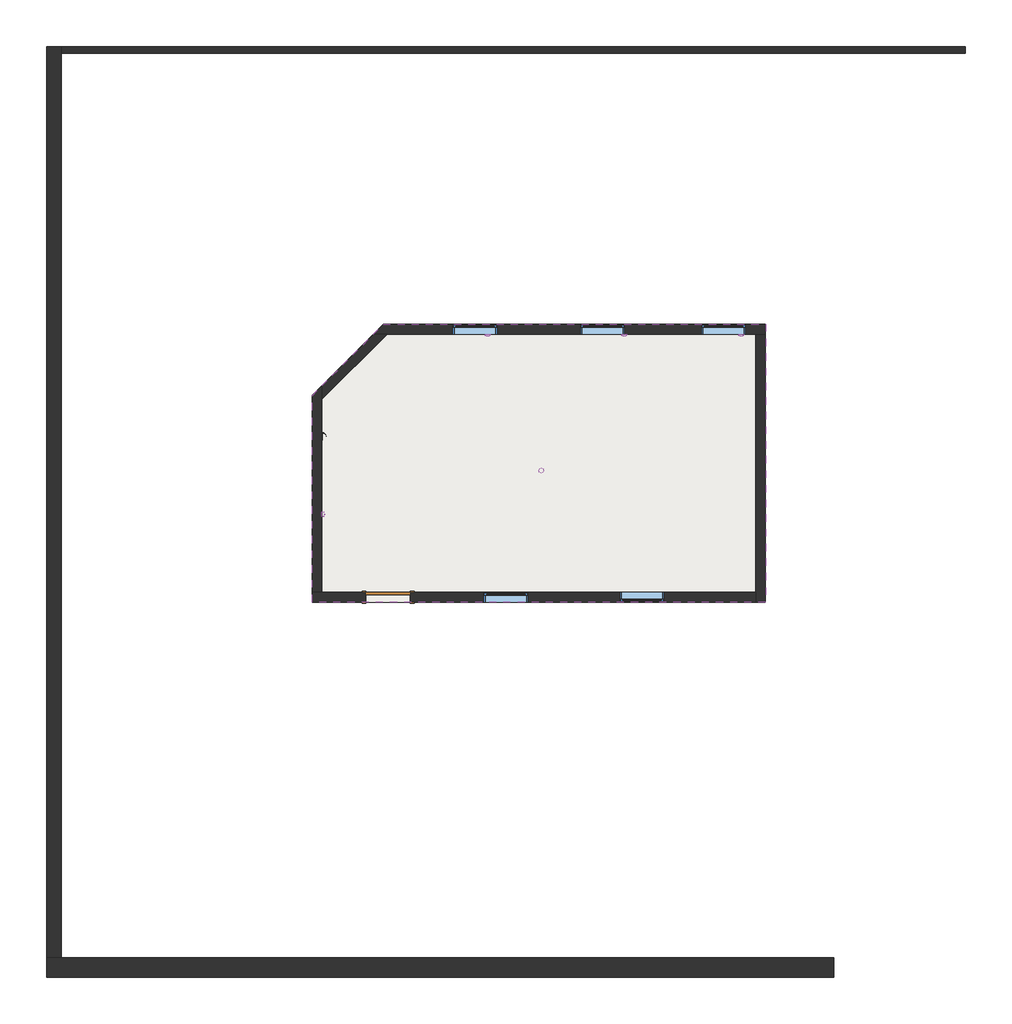
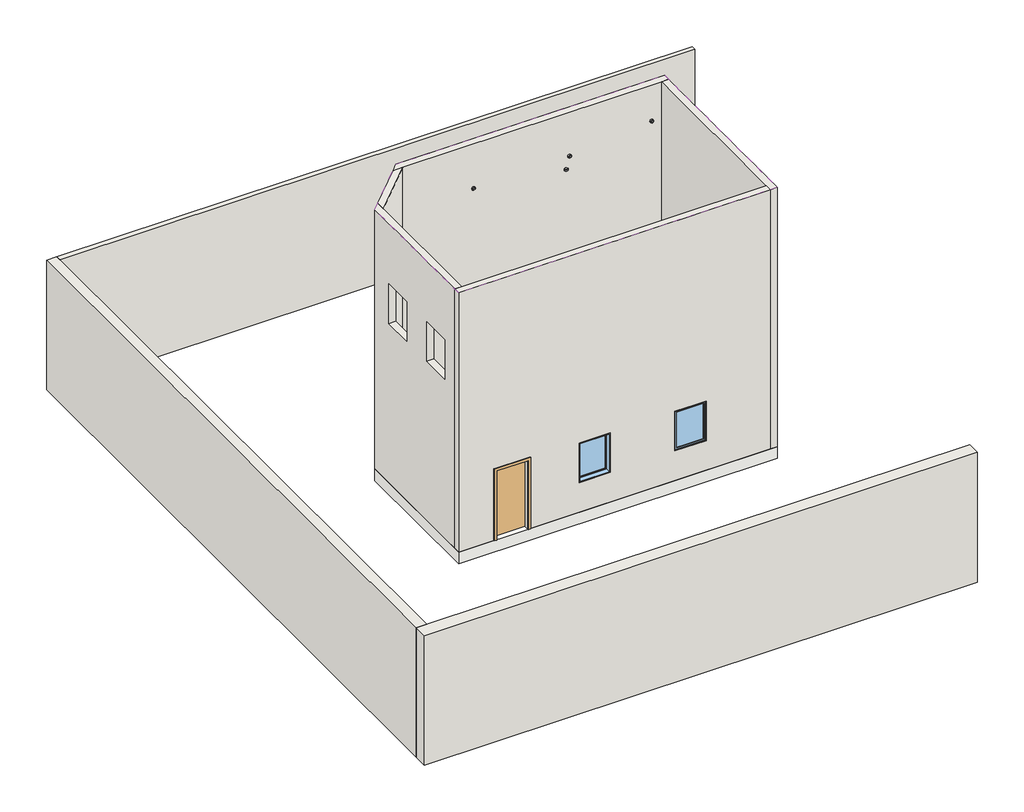
# One storey: 8 walls, 6 alarms, 5 windows, 1 door, 1 roof, 1 slab.
"""IFC4 building model written with IfcOpenShell, lengths in millimetres."""

import ifcopenshell
import ifcopenshell.guid

model = None  # the IFC model being written
_history = None  # IfcOwnerHistory: only IFC2X3 demands one
_inside = {}  # id of a spatial element -> (the spatial element, [elements in it])
_under = {}  # id of a project, library or spatial element -> (it, [spatial elements below it])
_declared = {}  # id of a project -> (the project, [libraries it declares])
_typed = {}  # id of a type object -> (the type object, [elements of that type])
_made_of = {}  # id of a material, layer set ... -> (it, [elements and type objects made of it])


def new_model(schema):
    """Start an empty IFC model of exactly this schema.

    Asked for "IFC4X3", IfcOpenShell would pick the latest addendum, in which some entities
    have other attributes; the version numbers below select the first issue.
    IFC2X3 requires an IfcOwnerHistory on every rooted entity: one is made here for all.
    """
    global model, _history
    if schema == "IFC4X3":
        model = ifcopenshell.file(schema_version=(4, 3, 0, 0))
    else:
        model = ifcopenshell.file(schema=schema)
    _inside.clear()
    _under.clear()
    _declared.clear()
    _typed.clear()
    _made_of.clear()
    _history = None
    if model.schema == "IFC2X3":
        org = make("IfcOrganization", Name="unknown")
        user = make(
            "IfcPersonAndOrganization",
            ThePerson=make("IfcPerson", FamilyName="unknown"),
            TheOrganization=org,
        )
        app = make(
            "IfcApplication",
            ApplicationDeveloper=org,
            Version="unknown",
            ApplicationFullName="unknown",
            ApplicationIdentifier="unknown",
        )
        _history = make(
            "IfcOwnerHistory",
            OwningUser=user,
            OwningApplication=app,
            ChangeAction="ADDED",
            CreationDate=0,
        )
    return model


def make(cls, **values):
    """One entity of the class cls with the attributes given. An attribute that is None is left unset."""
    return model.create_entity(
        cls, **{name: value for name, value in values.items() if value is not None}
    )


def rooted(cls, **values):
    """An entity with a GlobalId (a new one), such as an element, a storey or a relation."""
    return make(cls, GlobalId=ifcopenshell.guid.new(), OwnerHistory=_history, **values)


def si_unit(unit_type, name, prefix=None):
    """IfcSIUnit, for example si_unit("LENGTHUNIT", "METRE", prefix="MILLI")."""
    return make("IfcSIUnit", UnitType=unit_type, Prefix=prefix, Name=name)


def assignment(units):
    """IfcUnitAssignment: the units of a project."""
    return None if units is None else make("IfcUnitAssignment", Units=units)


def point(xyz):
    """IfcCartesianPoint."""
    return None if xyz is None else make("IfcCartesianPoint", Coordinates=xyz)


def direction(xyz):
    """IfcDirection."""
    return None if xyz is None else make("IfcDirection", DirectionRatios=xyz)


def frame(location, z_axis=None, x_axis=None):
    """IfcAxis2Placement3D, a coordinate frame: its origin and axes. An axis left out is left unset."""
    return make(
        "IfcAxis2Placement3D",
        Location=point(location),
        Axis=direction(z_axis),
        RefDirection=direction(x_axis),
    )


def frame_2d(location, x_axis=None):
    """IfcAxis2Placement2D, a coordinate frame in the plane: its origin and x axis."""
    return make(
        "IfcAxis2Placement2D", Location=point(location), RefDirection=direction(x_axis)
    )


def origin():
    """The frame at (0, 0, 0) with its axes left unset."""
    return frame((0.0, 0.0, 0.0))


def origin_with_axes():
    """The frame at (0, 0, 0) with the z axis (0, 0, 1) and the x axis (1, 0, 0) written out."""
    return frame((0.0, 0.0, 0.0), z_axis=(0.0, 0.0, 1.0), x_axis=(1.0, 0.0, 0.0))


def origin_2d():
    """The frame at (0, 0) in the plane with its x axis left unset."""
    return frame_2d((0.0, 0.0))


def place(relative_to, where):
    """IfcLocalPlacement: puts the frame where relative to a parent placement (None: the world)."""
    return make(
        "IfcLocalPlacement", PlacementRelTo=relative_to, RelativePlacement=where
    )


def context(
    kind, dimensions, precision=None, world=None, true_north=None, identifier=None
):
    """IfcGeometricRepresentationContext, for example the 3D "Model" context."""
    return make(
        "IfcGeometricRepresentationContext",
        ContextIdentifier=identifier,
        ContextType=kind,
        CoordinateSpaceDimension=dimensions,
        Precision=precision,
        WorldCoordinateSystem=world,
        TrueNorth=true_north,
    )


def project(units=None, contexts=None):
    """IfcProject with its units and contexts."""
    return rooted(
        "IfcProject",
        Name="project",
        RepresentationContexts=contexts,
        UnitsInContext=assignment(units),
    )


def spatial(cls, under=None, at=None, **own):
    """A site, building, storey or space (cls), placed at a placement, below another one or the project."""
    s = rooted(cls, ObjectPlacement=at, **own)
    if under is not None:
        _under.setdefault(under.id(), (under, []))[1].append(s)
    return s


def polyline(points):
    """IfcPolyline through the points."""
    return make("IfcPolyline", Points=[point(p) for p in points])


def circle_curve(where, radius):
    """IfcCircle in the frame where."""
    return make("IfcCircle", Position=where, Radius=radius)


def ellipse_curve(where, semi_axis1, semi_axis2):
    """IfcEllipse in the frame where."""
    return make(
        "IfcEllipse", Position=where, SemiAxis1=semi_axis1, SemiAxis2=semi_axis2
    )


def trimmed(basis, trim1, trim2, sense, master):
    """IfcTrimmedCurve: the piece of a basis curve between two trims."""
    return make(
        "IfcTrimmedCurve",
        BasisCurve=basis,
        Trim1=trim1,
        Trim2=trim2,
        SenseAgreement=sense,
        MasterRepresentation=master,
    )


def segment(curve, same_sense, transition):
    """IfcCompositeCurveSegment."""
    return make(
        "IfcCompositeCurveSegment",
        Transition=transition,
        SameSense=same_sense,
        ParentCurve=curve,
    )


def composite_curve(segments, self_intersect=None):
    """IfcCompositeCurve: segments joined end to end."""
    return make("IfcCompositeCurve", Segments=segments, SelfIntersect=self_intersect)


def outline(outer, holes=None, kind="AREA"):
    """IfcArbitraryClosedProfileDef: a profile drawn as a closed curve; with holes, ...WithVoids."""
    if holes is None:
        return make("IfcArbitraryClosedProfileDef", ProfileType=kind, OuterCurve=outer)
    return make(
        "IfcArbitraryProfileDefWithVoids",
        ProfileType=kind,
        OuterCurve=outer,
        InnerCurves=holes,
    )


def extrude(swept, where, along, depth):
    """IfcExtrudedAreaSolid: the profile swept, set in the frame where, extruded along a direction by depth."""
    return make(
        "IfcExtrudedAreaSolid",
        SweptArea=swept,
        Position=where,
        ExtrudedDirection=direction(along),
        Depth=depth,
    )


def faces_of(points, faces, orient=None, outer=None):
    """IfcFace entities. A face is a list of loops; a loop is a list of indices into points, from 0.

    orient and outer hold one flag for each loop. By default every Orientation is true, the
    first loop of a face is its IfcFaceOuterBound and the others are IfcFaceBound.
    """
    made = []
    for i, loops in enumerate(faces):
        bounds = []
        for j, loop in enumerate(loops):
            is_outer = j == 0 if outer is None else outer[i][j]
            bounds.append(
                make(
                    "IfcFaceOuterBound" if is_outer else "IfcFaceBound",
                    Bound=make("IfcPolyLoop", Polygon=[points[k] for k in loop]),
                    Orientation=True if orient is None else orient[i][j],
                )
            )
        made.append(make("IfcFace", Bounds=bounds))
    return made


def faceted_brep(points, faces, orient=None, outer=None, voids=None):
    """IfcFacetedBrep: a solid bounded by flat faces; with voids (closed shells), ...WithVoids."""
    shared = [point(p) for p in points]
    hull = make("IfcClosedShell", CfsFaces=faces_of(shared, faces, orient, outer))
    if voids is None:
        return make("IfcFacetedBrep", Outer=hull)
    return make(
        "IfcFacetedBrepWithVoids",
        Outer=hull,
        Voids=[
            make(cls, CfsFaces=faces_of(shared, fs, o, b)) for cls, fs, o, b in voids
        ],
    )


def shape(context_of_items, identifier, shape_type, items):
    """IfcShapeRepresentation: the items that make up one representation, for example the "Body"."""
    return make(
        "IfcShapeRepresentation",
        ContextOfItems=context_of_items,
        RepresentationIdentifier=identifier,
        RepresentationType=shape_type,
        Items=items,
    )


def source(mapping_origin, context_of_items, identifier, shape_type, items):
    """IfcRepresentationMap: a shape defined once, which mapped items show again and again."""
    return make(
        "IfcRepresentationMap",
        MappingOrigin=mapping_origin,
        MappedRepresentation=shape(context_of_items, identifier, shape_type, items),
    )


def transform(
    local_origin,
    x_axis=None,
    y_axis=None,
    z_axis=None,
    scale=None,
    scale2=None,
    scale3=None,
    uniform=True,
):
    """IfcCartesianTransformationOperator3D, or its non-uniform kind. x_axis, y_axis, z_axis: its Axis1, 2, 3."""
    if uniform:
        return make(
            "IfcCartesianTransformationOperator3D",
            Axis1=direction(x_axis),
            Axis2=direction(y_axis),
            LocalOrigin=point(local_origin),
            Scale=scale,
            Axis3=direction(z_axis),
        )
    return make(
        "IfcCartesianTransformationOperator3DnonUniform",
        Axis1=direction(x_axis),
        Axis2=direction(y_axis),
        LocalOrigin=point(local_origin),
        Scale=scale,
        Axis3=direction(z_axis),
        Scale2=scale2,
        Scale3=scale3,
    )


def mapped(mapping_source, mapping_target):
    """IfcMappedItem: shows the shape of a source again, moved by a transform."""
    return make(
        "IfcMappedItem", MappingSource=mapping_source, MappingTarget=mapping_target
    )


def made_of(thing, what):
    """Note that an element or type object is made of a material, layer set ...; save() writes the relation."""
    if what is not None:
        _made_of.setdefault(what.id(), (what, []))[1].append(thing)
    return thing


def element(
    cls,
    number,
    at=None,
    inside=None,
    cuts=None,
    type_object=None,
    material=None,
    context=None,
    identifier="Body",
    shape_type=None,
    held_by="IfcProductDefinitionShape",
    body=None,
    shapes=None,
    **own,
):
    """One element of the class cls, such as IfcWall. Its Tag is "e" and its number.

    at: its placement. inside: the storey or other place that contains it. cuts: it is an
    opening in that element (IfcRelVoidsElement). A single representation is given by context,
    identifier, shape_type and body (its items); several are given by shapes. held_by: the class
    of the entity that holds the representations. save() writes the other relations.
    """
    e = rooted(cls, Tag="e%d" % number, ObjectPlacement=at, **own)
    if body is not None:
        shapes = [shape(context, identifier, shape_type, body)]
    if shapes is not None:
        e.Representation = make(held_by, Representations=shapes)
    if inside is not None:
        _inside.setdefault(inside.id(), (inside, []))[1].append(e)
    if cuts is not None:
        rooted(
            "IfcRelVoidsElement", RelatingBuildingElement=cuts, RelatedOpeningElement=e
        )
    if type_object is not None:
        _typed.setdefault(type_object.id(), (type_object, []))[1].append(e)
    return made_of(e, material)


def aggregate(whole, parts):
    """IfcRelAggregates: a whole, such as a stair, and the parts it consists of."""
    return rooted("IfcRelAggregates", RelatingObject=whole, RelatedObjects=parts)


def save(model, path):
    """Write the relations noted so far, then the file.

    IfcRelAggregates (storeys below a building ...), IfcRelContainedInSpatialStructure (elements
    in a storey), IfcRelDefinesByType, IfcRelAssociatesMaterial and IfcRelDeclares: one each for
    every whole, place, type object, material and project.
    """
    for whole, parts in _under.values():
        aggregate(whole, parts)
    for where, things in _inside.values():
        rooted(
            "IfcRelContainedInSpatialStructure",
            RelatedElements=things,
            RelatingStructure=where,
        )
    for kind, things in _typed.values():
        rooted("IfcRelDefinesByType", RelatedObjects=things, RelatingType=kind)
    for what, things in _made_of.values():
        rooted("IfcRelAssociatesMaterial", RelatedObjects=things, RelatingMaterial=what)
    for by, libraries in _declared.values():
        rooted("IfcRelDeclares", RelatingContext=by, RelatedDefinitions=libraries)
    model.write(path)


def plane_surface(at):
    """IfcPlane: the flat surface through the origin of the frame at, square to its z axis."""
    return make("IfcPlane", Position=at)


def cylinder_surface(at, radius):
    """IfcCylindricalSurface: all points at the distance radius from the z axis of the frame at."""
    return make("IfcCylindricalSurface", Position=at, Radius=radius)


def revolved_surface(curve, axis_point, axis_direction):
    """IfcSurfaceOfRevolution: the curve turned about the line through axis_point along axis_direction."""
    return make(
        "IfcSurfaceOfRevolution",
        SweptCurve=make("IfcArbitraryOpenProfileDef", ProfileType="CURVE", Curve=curve),
        AxisPosition=make("IfcAxis1Placement", Location=point(axis_point), Axis=direction(axis_direction)),
    )


def advanced_brep(points, edges, surfaces, faces):
    """IfcAdvancedBrep: a solid bounded by faces that lie on surfaces and meet in shared edges.

    An edge is (start, end): straight between two places in points (the first is 0);
    or (start, end, curve); or (start, end, curve, False) where it runs against its curve.
    A face is (place in surfaces, loops), or (place, loops, False) where it looks against
    its surface's normal. A loop lists edges by number (the first is 1), with a minus sign
    where the edge is run from its end to its start. The first loop is the outer one.
    """
    corners = [point(p) for p in points]
    vertices = [make("IfcVertexPoint", VertexGeometry=c) for c in corners]
    made = []
    for start, end, *more in edges:
        made.append(
            make(
                "IfcEdgeCurve",
                EdgeStart=vertices[start],
                EdgeEnd=vertices[end],
                EdgeGeometry=more[0] if more else make("IfcPolyline", Points=[corners[start], corners[end]]),
                SameSense=more[1] if len(more) > 1 else True,
            )
        )
    hull = []
    for where, loops, *sense in faces:
        bounds = []
        for j, loop in enumerate(loops):
            ring = [make("IfcOrientedEdge", EdgeElement=made[abs(k) - 1], Orientation=k > 0) for k in loop]
            bounds.append(
                make(
                    "IfcFaceOuterBound" if j == 0 else "IfcFaceBound",
                    Bound=make("IfcEdgeLoop", EdgeList=ring),
                    Orientation=True,
                )
            )
        hull.append(make("IfcAdvancedFace", Bounds=bounds, FaceSurface=surfaces[where], SameSense=sense[0] if sense else True))
    return make("IfcAdvancedBrep", Outer=make("IfcClosedShell", CfsFaces=hull))


def alarm_29ba7a31(model_context):
    return source(origin(), model_context, "Body", "SolidModel", [
        advanced_brep(
        [(0.0, 0.0, 85.5), (76.0, 0.0, 9.5), (-76.0, 0.0, 9.5), (0.0, 0.0, 9.5)],
        [
            (0, 1, circle_curve(frame((0.0, 0.0, 9.5), z_axis=(0.0, 1.0, 0.0), x_axis=(1.0, 0.0, 0.0)), 76.0)),
            (1, 2, circle_curve(frame((0.0, 0.0, 9.5), z_axis=(0.0, 0.0, 1.0), x_axis=(1.0, 0.0, 0.0)), 76.0)),
            (2, 0, circle_curve(frame((0.0, 0.0, 9.5), z_axis=(0.0, 1.0, 0.0), x_axis=(-1.0, 0.0, 0.0)), 76.0)),
            (2, 1, circle_curve(frame((0.0, 0.0, 9.5), z_axis=(0.0, 0.0, 1.0), x_axis=(1.0, 0.0, 0.0)), 76.0)),
            (1, 3),
            (3, 2),
        ],
        [
            revolved_surface(trimmed(ellipse_curve(frame((0.0, 0.0, 9.5), z_axis=(0.0, -1.0, 0.0), x_axis=(1.0, 0.0, 0.0)), 76.0, 76.0), [point((76.0, 0.0, 9.5))], [point((0.0, 0.0, 85.5))], True, "CARTESIAN"), (0.0, 0.0, 2609.0581012), (0.0, 0.0, 1.0)),
            plane_surface(frame((0.0, 0.0, 9.5), z_axis=(0.0, 0.0, -1.0), x_axis=(1.0, 0.0, 0.0))),
        ],
        [
            (0, [[1, 2, 3]]),
            (0, [[-3, 4, -1]]),
            (1, [[-2, 5, 6]]),
            (1, [[-4, -6, -5]]),
        ],
    ),
        extrude(outline(composite_curve([segment(trimmed(circle_curve(origin_2d(), 76.0), [point((-76.0, 0.0))], [point((76.0, 0.0))], False, "CARTESIAN"), True, "CONTINUOUS"), segment(trimmed(circle_curve(origin_2d(), 76.0), [point((76.0, 0.0))], [point((-76.0, 0.0))], False, "CARTESIAN"), True, "CONTINUOUS")], self_intersect=False)), origin_with_axes(), (0.0, 0.0, 1.0), 9.5),
    ])


def alarm_53eb8f19(model_context):
    return source(origin(), model_context, "Body", "AdvancedBrep", [
        advanced_brep(
        [(52.0, 0.0, 0.0), (-52.0, 0.0, 0.0), (52.0, 0.0, 35.0), (-52.0, 0.0, 35.0), (-18.3847763, -18.3847763, 35.0), (0.0, 0.0, 35.0), (18.3847763, -18.3847763, 35.0), (0.0, 0.0, 60.0)],
        [
            (0, 1, circle_curve(frame((0.0, 0.0, 0.0), z_axis=(0.0, 0.0, -1.0), x_axis=(-1.0, 0.0, 0.0)), 52.0)),
            (1, 0, circle_curve(frame((0.0, 0.0, 0.0), z_axis=(0.0, 0.0, -1.0), x_axis=(-1.0, 0.0, 0.0)), 52.0)),
            (2, 3, circle_curve(frame((0.0, 0.0, 35.0), z_axis=(0.0, 0.0, 1.0), x_axis=(-1.0, 0.0, 0.0)), 52.0)),
            (3, 2, circle_curve(frame((0.0, 0.0, 35.0), z_axis=(0.0, 0.0, 1.0), x_axis=(-1.0, 0.0, 0.0)), 52.0)),
            (4, 5),
            (5, 6),
            (6, 4, circle_curve(frame((0.0, 0.0, 35.0), z_axis=(0.0, 0.0, -1.0), x_axis=(-0.7071067811865503, -0.7071067811865446, 0.0)), 26.0)),
            (1, 3),
            (2, 0),
            (4, 7),
            (7, 5),
            (7, 6),
        ],
        [
            plane_surface(frame((-52.0, 0.0, 0.0), z_axis=(0.0, 0.0, -1.0), x_axis=(0.0, 1.0, 0.0))),
            plane_surface(frame((-52.0, 0.0, 35.0), z_axis=(0.0, 0.0, 1.0), x_axis=(0.0, -1.0, 0.0))),
            cylinder_surface(frame((0.0, 0.0, 0.0), z_axis=(0.0, 0.0, 1.0), x_axis=(-1.0, 0.0, 0.0)), 52.0),
            plane_surface(frame((0.0, 0.0, 2609.0581012), z_axis=(-0.7071067811865447, 0.7071067811865505, 0.0), x_axis=(-0.7071067811865505, -0.7071067811865447, 0.0))),
            plane_surface(frame((0.0, 0.0, 2609.0581012), z_axis=(0.7071067811865515, 0.7071067811865437, 0.0), x_axis=(0.7071067811865437, -0.7071067811865515, 0.0))),
            revolved_surface(polyline([(-18.3847763, -18.3847763, 35.0), (0.0, 0.0, 60.0)]), (0.0, 0.0, 2609.0581012), (0.0, 0.0, 1.0)),
        ],
        [
            (0, [[1, 2]]),
            (1, [[3, 4], [5, 6, 7]]),
            (2, [[-2, 8, -3, 9]]),
            (2, [[-1, -9, -4, -8]]),
            (3, [[10, 11, -5]]),
            (4, [[-11, 12, -6]]),
            (5, [[-10, -7, -12]]),
        ],
    ),
        advanced_brep(
        [(26.0, 0.0, 35.0), (-26.0, 0.0, 35.0), (0.0, 0.0, 60.0), (0.0, 0.0, 35.0)],
        [
            (0, 1, circle_curve(frame((0.0, 0.0, 35.0), z_axis=(0.0, 0.0, 1.0), x_axis=(-1.0, 0.0, 0.0)), 26.0)),
            (1, 2),
            (2, 0),
            (1, 0, circle_curve(frame((0.0, 0.0, 35.0), z_axis=(0.0, 0.0, 1.0), x_axis=(-1.0, 0.0, 0.0)), 26.0)),
            (3, 1),
            (0, 3),
        ],
        [
            revolved_surface(polyline([(0.0, 0.0, 60.0), (-26.0, 0.0, 35.0)]), (0.0, 0.0, 2609.0581012), (0.0, 0.0, -1.0)),
            plane_surface(frame((0.0, 0.0, 35.0), z_axis=(0.0, 0.0, -1.0), x_axis=(-1.0, 0.0, 0.0))),
        ],
        [
            (0, [[1, 2, 3]]),
            (0, [[4, -3, -2]]),
            (1, [[5, -1, 6]]),
            (1, [[-6, -4, -5]]),
        ],
    ),
        advanced_brep(
        [(0.0, 0.0, 60.0), (-18.3847763, 18.3847763, 35.0), (0.0, 0.0, 35.0), (18.3847763, 18.3847763, 35.0)],
        [
            (0, 1),
            (1, 2),
            (2, 0),
            (2, 3),
            (3, 0),
            (1, 3, circle_curve(frame((0.0, 0.0, 35.0), z_axis=(0.0, 0.0, -1.0), x_axis=(-0.707106781186547, 0.7071067811865482, 0.0)), 26.0)),
        ],
        [
            plane_surface(frame((0.0, 0.0, 2343.8067943), z_axis=(-0.7071067811865482, -0.707106781186547, 0.0), x_axis=(-0.707106781186547, 0.7071067811865482, 0.0))),
            plane_surface(frame((0.0, 0.0, 2343.8067943), z_axis=(0.7071067811865482, -0.707106781186547, 0.0), x_axis=(0.707106781186547, 0.7071067811865482, 0.0))),
            plane_surface(frame((0.0, 0.0, 35.0), z_axis=(0.0, 0.0, -1.0000000000000002), x_axis=(-0.707106781186547, 0.7071067811865482, 0.0))),
            revolved_surface(polyline([(-18.3847763, 18.3847763, 35.0), (0.0, 0.0, 60.0)]), (0.0, 0.0, 2343.8067943), (0.0, 0.0, 1.0)),
        ],
        [
            (0, [[1, 2, 3]]),
            (1, [[4, 5, -3]]),
            (2, [[-2, 6, -4]]),
            (3, [[-6, -1, -5]]),
        ],
    ),
        advanced_brep(
        [(0.0, 0.0, 60.0), (0.0, 0.0, 35.0), (-18.3847763, 18.3847763, 35.0), (-18.3847763, -18.3847763, 35.0)],
        [
            (0, 1),
            (1, 2),
            (2, 0),
            (0, 3),
            (3, 1),
            (3, 2, circle_curve(frame((0.0, 0.0, 35.0), z_axis=(0.0, 0.0, -1.0), x_axis=(-0.707106781186547, 0.7071067811865482, 0.0)), 26.0)),
        ],
        [
            plane_surface(frame((0.0, 0.0, 2343.8067943), z_axis=(0.7071067811865482, 0.707106781186547, 0.0), x_axis=(-0.707106781186547, 0.7071067811865482, 0.0))),
            plane_surface(frame((0.0, 0.0, 2343.8067943), z_axis=(0.7071067811865459, -0.7071067811865491, 0.0), x_axis=(-0.7071067811865491, -0.7071067811865459, 0.0))),
            plane_surface(frame((0.0, 0.0, 35.0), z_axis=(0.0, 0.0, -1.0000000000000002), x_axis=(-0.707106781186547, 0.7071067811865482, 0.0))),
            revolved_surface(polyline([(-18.3847763, 18.3847763, 35.0), (0.0, 0.0, 60.0)]), (0.0, 0.0, 2343.8067943), (0.0, 0.0, 1.0)),
        ],
        [
            (0, [[1, 2, 3]]),
            (1, [[4, 5, -1]]),
            (2, [[6, -2, -5]]),
            (3, [[-3, -6, -4]]),
        ],
    ),
        advanced_brep(
        [(18.3847763, -18.3847763, 35.0), (0.0, 0.0, 60.0), (0.0, 0.0, 35.0), (18.3847763, 18.3847763, 35.0)],
        [
            (0, 1),
            (1, 2),
            (2, 0),
            (3, 2),
            (1, 3),
            (0, 3, circle_curve(frame((0.0, 0.0, 35.0), z_axis=(0.0, 0.0, 1.0), x_axis=(0.7071067811865503, -0.7071067811865446, 0.0)), 26.0)),
        ],
        [
            plane_surface(frame((0.0, 0.0, 2609.0581012), z_axis=(-0.7071067811865447, -0.7071067811865505, 0.0), x_axis=(0.7071067811865505, -0.7071067811865447, 0.0))),
            plane_surface(frame((0.0, 0.0, 2609.0581012), z_axis=(-0.7071067811865491, 0.707106781186546, 0.0), x_axis=(0.707106781186546, 0.7071067811865491, 0.0))),
            revolved_surface(polyline([(0.0, 0.0, 60.0), (18.3847763, -18.3847763, 35.0)]), (0.0, 0.0, 2609.0581012), (0.0, 0.0, -1.0)),
            plane_surface(frame((0.0, 0.0, 35.0), z_axis=(0.0, 0.0, -1.0), x_axis=(0.7071067811865505, -0.7071067811865447, 0.0))),
        ],
        [
            (0, [[1, 2, 3]]),
            (1, [[4, -2, 5]]),
            (2, [[-1, 6, -5]]),
            (3, [[-6, -3, -4]]),
        ],
    ),
    ])


def alarm_5285ee31(model_context):
    return source(origin(), model_context, "Body", "AdvancedBrep", [
        advanced_brep(
        [(-26.0, 0.0, 50.0), (26.0, 0.0, 50.0), (-52.0, 0.0, 0.0), (52.0, 0.0, 0.0), (-26.0, 0.0, 35.0), (26.0, 0.0, 35.0), (-52.0, 0.0, 35.0), (52.0, 0.0, 35.0)],
        [
            (0, 1, circle_curve(frame((0.0, 0.0, 50.0), z_axis=(0.0, 0.0, 1.0), x_axis=(1.0, 0.0, 0.0)), 26.0)),
            (1, 0, circle_curve(frame((0.0, 0.0, 50.0), z_axis=(0.0, 0.0, 1.0), x_axis=(1.0, 0.0, 0.0)), 26.0)),
            (2, 3, circle_curve(frame((0.0, 0.0, 0.0), z_axis=(0.0, 0.0, -1.0), x_axis=(1.0, 0.0, 0.0)), 52.0)),
            (3, 2, circle_curve(frame((0.0, 0.0, 0.0), z_axis=(0.0, 0.0, -1.0), x_axis=(1.0, 0.0, 0.0)), 52.0)),
            (0, 4),
            (4, 5, circle_curve(frame((0.0, 0.0, 35.0), z_axis=(0.0, 0.0, 1.0), x_axis=(1.0, 0.0, 0.0)), 26.0)),
            (5, 1),
            (5, 4, circle_curve(frame((0.0, 0.0, 35.0), z_axis=(0.0, 0.0, 1.0), x_axis=(1.0, 0.0, 0.0)), 26.0)),
            (6, 7, circle_curve(frame((0.0, 0.0, 35.0), z_axis=(0.0, 0.0, 1.0), x_axis=(1.0, 0.0, 0.0)), 52.0)),
            (7, 6, circle_curve(frame((0.0, 0.0, 35.0), z_axis=(0.0, 0.0, 1.0), x_axis=(1.0, 0.0, 0.0)), 52.0)),
            (3, 7),
            (6, 2),
        ],
        [
            plane_surface(frame((26.0, 0.0, 50.0), z_axis=(0.0, 0.0, 1.0), x_axis=(0.0, 1.0, 0.0))),
            plane_surface(frame((26.0, 0.0, 0.0), z_axis=(0.0, 0.0, -1.0), x_axis=(0.0, -1.0, 0.0))),
            cylinder_surface(origin_with_axes(), 26.0),
            plane_surface(frame((52.0, 0.0, 35.0), z_axis=(0.0, 0.0, 1.0), x_axis=(0.0, 1.0, 0.0))),
            cylinder_surface(origin_with_axes(), 52.0),
        ],
        [
            (0, [[1, 2]]),
            (1, [[3, 4]]),
            (2, [[-1, 5, 6, 7]]),
            (2, [[-2, -7, 8, -5]]),
            (3, [[9, 10], [-6, -8]]),
            (4, [[-4, 11, -9, 12]]),
            (4, [[-3, -12, -10, -11]]),
        ],
    ),
    ])


def door_0915_x_2134mm_6a9e8738(model_context):
    return source(origin(), model_context, "Body", "SweptSolid", [
        extrude(outline(polyline([(2210.0, -533.5), (0.0, -533.5), (0.0, -457.5), (2134.0, -457.5), (2134.0, 457.5), (0.0, 457.5), (0.0, 533.5), (2210.0, 533.5), (2210.0, -533.5)])), frame((0.0, 100.0, 0.0), z_axis=(0.0, 1.0, 0.0), x_axis=(0.0, 0.0, 1.0)), (0.0, 0.0, 1.0), 25.0),
        extrude(outline(polyline([(2210.0, 533.5), (2210.0, -533.5), (0.0, -533.5), (0.0, -457.5), (2134.0, -457.5), (2134.0, 457.5), (0.0, 457.5), (0.0, 533.5), (2210.0, 533.5)])), frame((0.0, -125.0, 0.0), z_axis=(0.0, 1.0, 0.0), x_axis=(0.0, 0.0, 1.0)), (0.0, 0.0, 1.0), 25.0),
        extrude(outline(polyline([(457.5, 49.0), (-457.5, 49.0), (-457.5, 100.0), (457.5, 100.0), (457.5, 49.0)])), origin_with_axes(), (0.0, 0.0, 1.0), 2134.0),
    ])


def window_0915_x_1220mm_488fb2fb(model_context):
    return source(origin(), model_context, "Body", "SweptSolid", [
        extrude(outline(polyline([(-394.5, 78.0), (394.5, 78.0), (394.5, 66.0), (-394.5, 66.0), (-394.5, 78.0)])), frame((0.0, 0.0, 978.0), z_axis=(0.0, 0.0, 1.0), x_axis=(1.0, 0.0, 0.0)), (0.0, 0.0, 1.0), 1094.0),
        extrude(outline(polyline([(2116.0, -438.5), (934.0, -438.5), (934.0, 438.5), (2116.0, 438.5), (2116.0, -438.5)]), holes=[polyline([(2072.0, -394.5), (2072.0, 394.5), (978.0, 394.5), (978.0, -394.5), (2072.0, -394.5)])]), frame((0.0, 50.0, 0.0), z_axis=(0.0, 1.0, 0.0), x_axis=(0.0, 0.0, 1.0)), (0.0, 0.0, 1.0), 44.0),
        extrude(outline(polyline([(2135.0, -457.5), (915.0, -457.5), (915.0, 457.5), (2135.0, 457.5), (2135.0, -457.5)]), holes=[polyline([(2116.0, -438.5), (2116.0, 438.5), (934.0, 438.5), (934.0, -438.5), (2116.0, -438.5)])]), frame((0.0, 50.0, 0.0), z_axis=(0.0, 1.0, 0.0), x_axis=(0.0, 0.0, 1.0)), (0.0, 0.0, 1.0), 63.0),
        extrude(outline(polyline([(2135.0, -457.5), (915.0, -457.5), (915.0, 457.5), (2135.0, 457.5), (2135.0, -457.5)]), holes=[polyline([(2103.0, -425.5), (2103.0, 425.5), (947.0, 425.5), (947.0, -425.5), (2103.0, -425.5)])]), frame((0.0, -87.0, 0.0), z_axis=(0.0, 1.0, 0.0), x_axis=(0.0, 0.0, 1.0)), (0.0, 0.0, 1.0), 137.0),
    ])


model = new_model("IFC4")

# Units and contexts
model_context = context("Model", 3, world=origin())
ifc_project = project(units=[si_unit("LENGTHUNIT", "METRE", prefix="MILLI")], contexts=[model_context])

# Site, building, storey
site = spatial("IfcSite", under=ifc_project)
building = spatial("IfcBuilding", under=site)
storey = spatial("IfcBuildingStorey", under=building, Name="标高 1", Elevation=0.0)

# Alarms
placement = place(None, origin())
alarm_shape = alarm_29ba7a31(model_context)
element("IfcAlarm", 1, ObjectType="报警闪灯 : 标准", at=placement, inside=storey, context=model_context, shape_type="MappedRepresentation", body=[
    mapped(alarm_shape, transform((-7480.1449608, 2535.4590579, 1200.0), x_axis=(0.0, 1.0, 0.0), y_axis=(0.0, 0.0, 1.0), z_axis=(1.0, 0.0, 0.0))),
])
alarm_2_shape = alarm_53eb8f19(model_context)
element("IfcAlarm", 2, ObjectType="电子感温探测器 : 防爆型", at=placement, inside=storey, context=model_context, shape_type="MappedRepresentation", body=[
    mapped(alarm_2_shape, transform((-7480.1449608, 935.4590579, 6895.7404718), x_axis=(0.0, 1.0, 0.0), y_axis=(0.0, 0.0, 1.0), z_axis=(1.0, 0.0, 0.0))),
])
alarm_3_shape = alarm_5285ee31(model_context)
element("IfcAlarm", 3, ObjectType="光电感烟探测器 : 点型", at=placement, inside=storey, context=model_context, shape_type="MappedRepresentation", body=[
    mapped(alarm_3_shape, transform((-2980.1449608, 1835.4590579, 8508.5629281), x_axis=(1.0, 0.0, 0.0), y_axis=(0.0, 1.0, 0.0), z_axis=(0.0, 0.0, 1.0))),
])
element("IfcAlarm", 4, ObjectType="光电感烟探测器 : 点型", at=placement, inside=storey, context=model_context, shape_type="MappedRepresentation", body=[
    mapped(alarm_3_shape, transform((-4080.1449608, 4635.4590579, 6642.6361081), x_axis=(1.0, 0.0, 0.0), y_axis=(0.0, 0.0, 1.0), z_axis=(0.0, -1.0, 0.0))),
])
element("IfcAlarm", 5, ObjectType="光电感烟探测器 : 点型", at=placement, inside=storey, context=model_context, shape_type="MappedRepresentation", body=[
    mapped(alarm_3_shape, transform((-1280.1449608, 4635.4590579, 6660.302945), x_axis=(1.0, 0.0, 0.0), y_axis=(0.0, 0.0, 1.0), z_axis=(0.0, -1.0, 0.0))),
])
element("IfcAlarm", 6, ObjectType="光电感烟探测器 : 点型", at=placement, inside=storey, context=model_context, shape_type="MappedRepresentation", body=[
    mapped(alarm_3_shape, transform((1119.8550392, 4635.4590579, 6900.0711466), x_axis=(1.0, 0.0, 0.0), y_axis=(0.0, 0.0, 1.0), z_axis=(0.0, -1.0, 0.0))),
])

# Door
door_0915_x_2134mm_shape = door_0915_x_2134mm_6a9e8738(model_context)
element("IfcDoor", 7, ObjectType="单扇 - 与墙齐 : 0915 x 2134mm", at=placement, inside=storey, context=model_context, shape_type="MappedRepresentation", body=[
    mapped(door_0915_x_2134mm_shape, transform((-6122.6449608, -764.5409421, 0.0), x_axis=(1.0, 0.0, 0.0), y_axis=(0.0, 1.0, 0.0), z_axis=(0.0, 0.0, 1.0))),
])

# Roof
element("IfcRoof", 8, ObjectType="钢筋托梁 - 钢面板 - EPDM 薄膜", at=placement, inside=storey, context=model_context, shape_type="SweptSolid", body=[
    extrude(outline(polyline([(-7683.1449608, 3373.8804141), (-6218.566317, 4838.4590579), (1622.8550392, 4838.4590579), (1622.8550392, -867.5409421), (-7683.1449608, -867.5409421), (-7683.1449608, 3373.8804141)])), frame((0.0, 0.0, 8003.5629281), z_axis=(0.0, 0.0, 1.0), x_axis=(1.0, 0.0, 0.0)), (0.0, 0.0, 1.0), 505.0),
])

# Slab
element("IfcSlab", 9, ObjectType="混凝土 - 商用 362mm", at=placement, inside=storey, context=model_context, shape_type="SweptSolid", body=[
    extrude(outline(polyline([(-6221.566317, 4835.4590579), (1619.8550392, 4835.4590579), (1619.8550392, -864.5409421), (-7680.1449608, -864.5409421), (-7680.1449608, 3376.8804141), (-6221.566317, 4835.4590579)])), frame((0.0, 0.0, -362.0), z_axis=(0.0, 0.0, 1.0), x_axis=(1.0, 0.0, 0.0)), (0.0, 0.0, 1.0), 362.0),
])

# Walls
element("IfcWall", 10, ObjectType="常规 - 200mm", at=placement, inside=storey, context=model_context, shape_type="Brep", body=[
    faceted_brep([(-6421.566317, 4635.4590579, 0.0), (-6138.7236046, 4635.4590579, 0.0), (1419.8550392, 4635.4590579, 0.0), (1619.8550392, 4635.4590579, 0.0), (1619.8550392, 4635.4590579, 8000.0), (1419.8550392, 4635.4590579, 8000.0), (-6138.7236046, 4635.4590579, 8000.0), (-6421.566317, 4635.4590579, 8000.0), (-4795.1449608, 4635.4590579, 915.0), (-4795.1449608, 4635.4590579, 2135.0), (-3880.1449608, 4635.4590579, 2135.0), (-3880.1449608, 4635.4590579, 915.0), (-2180.1449608, 4635.4590579, 915.0), (-2180.1449608, 4635.4590579, 2135.0), (-1265.1449608, 4635.4590579, 2135.0), (-1265.1449608, 4635.4590579, 915.0), (304.8550392, 4635.4590579, 915.0), (304.8550392, 4635.4590579, 2135.0), (1219.8550392, 4635.4590579, 2135.0), (1219.8550392, 4635.4590579, 915.0), (1619.8550392, 4835.4590579, 0.0), (-6221.566317, 4835.4590579, 0.0), (-6221.566317, 4835.4590579, 8000.0), (1619.8550392, 4835.4590579, 8000.0), (-4795.1449608, 4835.4590579, 915.0), (-3880.1449608, 4835.4590579, 915.0), (-3880.1449608, 4835.4590579, 2135.0), (-4795.1449608, 4835.4590579, 2135.0), (-2180.1449608, 4835.4590579, 915.0), (-1265.1449608, 4835.4590579, 915.0), (-1265.1449608, 4835.4590579, 2135.0), (-2180.1449608, 4835.4590579, 2135.0), (304.8550392, 4835.4590579, 2135.0), (304.8550392, 4835.4590579, 915.0), (1219.8550392, 4835.4590579, 915.0), (1219.8550392, 4835.4590579, 2135.0)], [[[0, 1, 2, 3, 4, 5, 6, 7], [8, 9, 10, 11], [12, 13, 14, 15], [16, 17, 18, 19]], [[20, 21, 22, 23], [24, 25, 26, 27], [28, 29, 30, 31], [32, 33, 34, 35]], [[3, 2, 1, 0, 21, 20]], [[7, 6, 5, 4, 23, 22]], [[4, 3, 20, 23]], [[0, 7, 22, 21]], [[9, 8, 24, 27]], [[10, 9, 27, 26]], [[11, 10, 26, 25]], [[8, 11, 25, 24]], [[13, 12, 28, 31]], [[14, 13, 31, 30]], [[15, 14, 30, 29]], [[12, 15, 29, 28]], [[16, 33, 32, 17]], [[17, 32, 35, 18]], [[18, 35, 34, 19]], [[33, 16, 19, 34]]]),
])
element("IfcWall", 11, ObjectType="常规 - 200mm", at=placement, inside=storey, context=model_context, shape_type="Brep", body=[
    faceted_brep([(1419.8550392, 4635.4590579, 0.0), (1419.8550392, -664.5409421, 0.0), (1419.8550392, -864.5409421, 0.0), (1419.8550392, -864.5409421, 8000.0), (1419.8550392, -664.5409421, 8000.0), (1419.8550392, 4635.4590579, 8000.0), (1619.8550392, 4635.4590579, 0.0), (1619.8550392, 4635.4590579, 8000.0), (1619.8550392, -864.5409421, 8000.0), (1619.8550392, -864.5409421, 0.0)], [[[0, 1, 2, 3, 4, 5]], [[6, 7, 8, 9]], [[2, 1, 0, 6, 9]], [[5, 4, 3, 8, 7]], [[0, 5, 7, 6]], [[3, 2, 9, 8]]]),
])
element("IfcWall", 12, ObjectType="常规 - 200mm", at=placement, inside=storey, context=model_context, shape_type="Brep", body=[
    faceted_brep([(1419.8550392, -664.5409421, 0.0), (-5665.1449608, -664.5409421, 0.0), (-5665.1449608, -664.5409421, 2134.0), (-6580.1449608, -664.5409421, 2134.0), (-6580.1449608, -664.5409421, 0.0), (-7480.1449608, -664.5409421, 0.0), (-7680.1449608, -664.5409421, 0.0), (-7680.1449608, -664.5409421, 8000.0), (-7480.1449608, -664.5409421, 8000.0), (1419.8550392, -664.5409421, 8000.0), (-4165.1449608, -664.5409421, 915.0), (-3250.1449608, -664.5409421, 915.0), (-3250.1449608, -664.5409421, 2135.0), (-4165.1449608, -664.5409421, 2135.0), (-457.6449608, -664.5409421, 915.0), (-457.6449608, -664.5409421, 2135.0), (-1372.6449608, -664.5409421, 2135.0), (-1372.6449608, -664.5409421, 915.0), (-5665.1449608, -864.5409421, 2134.0), (-5665.1449608, -864.5409421, 0.0), (1419.8550392, -864.5409421, 0.0), (1419.8550392, -864.5409421, 8000.0), (-7680.1449608, -864.5409421, 8000.0), (-7680.1449608, -864.5409421, 0.0), (-6580.1449608, -864.5409421, 0.0), (-6580.1449608, -864.5409421, 2134.0), (-4165.1449608, -864.5409421, 915.0), (-4165.1449608, -864.5409421, 2135.0), (-3250.1449608, -864.5409421, 2135.0), (-3250.1449608, -864.5409421, 915.0), (-457.6449608, -864.5409421, 2135.0), (-457.6449608, -864.5409421, 915.0), (-1372.6449608, -864.5409421, 915.0), (-1372.6449608, -864.5409421, 2135.0)], [[[0, 1, 2, 3, 4, 5, 6, 7, 8, 9], [10, 11, 12, 13], [14, 15, 16, 17]], [[18, 19, 20, 21, 22, 23, 24, 25], [26, 27, 28, 29], [30, 31, 32, 33]], [[24, 23, 6, 5, 4]], [[20, 19, 1, 0]], [[9, 8, 7, 22, 21]], [[0, 9, 21, 20]], [[7, 6, 23, 22]], [[2, 1, 19, 18]], [[3, 2, 18, 25]], [[4, 3, 25, 24]], [[27, 26, 10, 13]], [[28, 27, 13, 12]], [[29, 28, 12, 11]], [[26, 29, 11, 10]], [[14, 31, 30, 15]], [[15, 30, 33, 16]], [[16, 33, 32, 17]], [[31, 14, 17, 32]]]),
])
element("IfcWall", 13, ObjectType="常规 - 200mm", at=placement, inside=storey, context=model_context, shape_type="Brep", body=[
    faceted_brep([(-7480.1449608, -664.5409421, 0.0), (-7480.1449608, 3294.0377016, 0.0), (-7480.1449608, 3576.8804141, 0.0), (-7480.1449608, 3576.8804141, 8000.0), (-7480.1449608, 3294.0377016, 8000.0), (-7480.1449608, -664.5409421, 8000.0), (-7480.1449608, -164.5409421, 4915.0), (-7480.1449608, -164.5409421, 6135.0), (-7480.1449608, 750.4590579, 6135.0), (-7480.1449608, 750.4590579, 4915.0), (-7480.1449608, 1750.4590579, 4915.0), (-7480.1449608, 1750.4590579, 6135.0), (-7480.1449608, 2665.4590579, 6135.0), (-7480.1449608, 2665.4590579, 4915.0), (-7680.1449608, -664.5409421, 0.0), (-7680.1449608, -664.5409421, 8000.0), (-7680.1449608, 3376.8804141, 8000.0), (-7680.1449608, 3376.8804141, 0.0), (-7680.1449608, -164.5409421, 4915.0), (-7680.1449608, 750.4590579, 4915.0), (-7680.1449608, 750.4590579, 6135.0), (-7680.1449608, -164.5409421, 6135.0), (-7680.1449608, 1750.4590579, 4915.0), (-7680.1449608, 2665.4590579, 4915.0), (-7680.1449608, 2665.4590579, 6135.0), (-7680.1449608, 1750.4590579, 6135.0)], [[[0, 1, 2, 3, 4, 5], [6, 7, 8, 9], [10, 11, 12, 13]], [[14, 15, 16, 17], [18, 19, 20, 21], [22, 23, 24, 25]], [[2, 1, 0, 14, 17]], [[5, 4, 3, 16, 15]], [[0, 5, 15, 14]], [[3, 2, 17, 16]], [[7, 6, 18, 21]], [[8, 7, 21, 20]], [[9, 8, 20, 19]], [[6, 9, 19, 18]], [[11, 10, 22, 25]], [[12, 11, 25, 24]], [[13, 12, 24, 23]], [[10, 13, 23, 22]]]),
])
element("IfcWall", 14, ObjectType="常规 - 200mm", at=placement, inside=storey, context=model_context, shape_type="SweptSolid", body=[
    extrude(outline(polyline([(-6138.7236046, 4635.4590579), (-7480.1449608, 3294.0377016), (-7480.1449608, 3576.8804141), (-6421.566317, 4635.4590579), (-6138.7236046, 4635.4590579)])), origin_with_axes(), (0.0, 0.0, 1.0), 8000.0),
])
element("IfcWall", 15, ObjectType="常规 - 140mm 砌体", at=placement, inside=storey, context=model_context, shape_type="SweptSolid", body=[
    extrude(outline(polyline([(5719.8550392, 10395.4590579), (-12830.1449608, 10395.4590579), (-12830.1449608, 10535.4590579), (5719.8550392, 10535.4590579), (5719.8550392, 10395.4590579)])), origin_with_axes(), (0.0, 0.0, 1.0), 4000.0),
])
element("IfcWall", 16, ObjectType="常规 - 225mm 砌体", at=placement, inside=storey, context=model_context, shape_type="Brep", body=[
    faceted_brep([(3019.8550392, -8164.5409421, 0.0), (-12830.1449608, -8164.5409421, 0.0), (-13130.1449608, -8164.5409421, 0.0), (-13130.1449608, -8164.5409421, 4000.0), (-12830.1449608, -8164.5409421, 4000.0), (3019.8550392, -8164.5409421, 4000.0), (3019.8550392, -8564.5409421, 0.0), (3019.8550392, -8564.5409421, 4000.0), (-13130.1449608, -8564.5409421, 4000.0), (-13130.1449608, -8564.5409421, 0.0)], [[[0, 1, 2, 3, 4, 5]], [[6, 7, 8, 9]], [[3, 2, 9, 8]], [[2, 1, 0, 6, 9]], [[5, 4, 3, 8, 7]], [[0, 5, 7, 6]]]),
])
element("IfcWall", 17, ObjectType="挡土墙 - 300mm 混凝土", at=placement, inside=storey, context=model_context, shape_type="Brep", body=[
    faceted_brep([(-12830.1449608, -8164.5409421, 0.0), (-12830.1449608, 10395.4590579, 0.0), (-12830.1449608, 10535.4590579, 0.0), (-12830.1449608, 10535.4590579, 4000.0), (-12830.1449608, 10395.4590579, 4000.0), (-12830.1449608, -8164.5409421, 4000.0), (-13130.1449608, -8164.5409421, 0.0), (-13130.1449608, -8164.5409421, 4000.0), (-13130.1449608, 10535.4590579, 4000.0), (-13130.1449608, 10535.4590579, 0.0)], [[[0, 1, 2, 3, 4, 5]], [[6, 7, 8, 9]], [[0, 5, 7, 6]], [[2, 1, 0, 6, 9]], [[5, 4, 3, 8, 7]], [[3, 2, 9, 8]]]),
])

# Windows
window_0915_x_1220mm_shape = window_0915_x_1220mm_488fb2fb(model_context)
element("IfcWindow", 18, ObjectType="固定 : 0915 x 1220mm", at=placement, inside=storey, context=model_context, shape_type="MappedRepresentation", body=[
    mapped(window_0915_x_1220mm_shape, transform((-3707.6449608, -777.5409421, 0.0), x_axis=(1.0, 0.0, 0.0), y_axis=(0.0, 1.0, 0.0), z_axis=(0.0, 0.0, 1.0))),
])
element("IfcWindow", 19, ObjectType="固定 : 0915 x 1220mm", at=placement, inside=storey, context=model_context, shape_type="MappedRepresentation", body=[
    mapped(window_0915_x_1220mm_shape, transform((-915.1449608, -751.5409421, 0.0), x_axis=(-1.0, 0.0, 0.0), y_axis=(0.0, -1.0, 0.0), z_axis=(0.0, 0.0, 1.0))),
])
element("IfcWindow", 20, ObjectType="固定 : 0915 x 1220mm", at=placement, inside=storey, context=model_context, shape_type="MappedRepresentation", body=[
    mapped(window_0915_x_1220mm_shape, transform((-4337.6449608, 4722.4590579, 0.0), x_axis=(1.0, 0.0, 0.0), y_axis=(0.0, 1.0, 0.0), z_axis=(0.0, 0.0, 1.0))),
])
element("IfcWindow", 21, ObjectType="固定 : 0915 x 1220mm", at=placement, inside=storey, context=model_context, shape_type="MappedRepresentation", body=[
    mapped(window_0915_x_1220mm_shape, transform((-1722.6449608, 4722.4590579, 0.0), x_axis=(1.0, 0.0, 0.0), y_axis=(0.0, 1.0, 0.0), z_axis=(0.0, 0.0, 1.0))),
])
element("IfcWindow", 22, ObjectType="固定 : 0915 x 1220mm", at=placement, inside=storey, context=model_context, shape_type="MappedRepresentation", body=[
    mapped(window_0915_x_1220mm_shape, transform((762.3550392, 4722.4590579, 0.0), x_axis=(1.0, 0.0, 0.0), y_axis=(0.0, 1.0, 0.0), z_axis=(0.0, 0.0, 1.0))),
])

save(model, "model.ifc")

# Revit data of these elements
# Project information
#   项目发布日期 = "出图日期"
#   项目状态 = "项目状态"
#   客户姓名 = "所有者"
#   项目地址 = "请在此处输入地址"
#   项目名称 = "项目名称"
#   项目编号 = "项目编号"
# Type "报警闪灯 : 标准"
#   半径 = 76 mm
#   高度 = 9.5 mm
#   直径 = 152 mm
#   Default Elevation = 1200 mm
#   材质 = none
# Type "电子感温探测器 : 防爆型"
#   半径 2 = 52 mm
#   半径 1 = 26 mm
#   长度 3 = 18.385 mm
#   长度 2 = 22.517 mm
#   长度 1 = 36.77 mm
#   高度 4 = 1.562 mm
#   高度 3 = 17.5 mm
#   高度 2 = 25 mm
#   高度 1 = 35 mm
#   Default Elevation = 1200 mm
#   可见性 1 = no
#   可见性 2 = yes
#   材质 = none
# Type "光电感烟探测器 : 点型"
#   半径 3 = 36.77 mm
#   半径 2 = 52 mm
#   半径 1 = 26 mm
#   高度 2 = 15 mm
#   高度 1 = 35 mm
#   Default Elevation = 1200 mm
#   可见性 2 = no
#   可见性 1 = yes
#   材质 = none
# Type "单扇 - 与墙齐 : 0915 x 2134mm"
#   Type Mark = "10"
#   Construction Type Id = "MDOOR"
#   Analytic Construction = "金属"
#   Thickness = 51 mm
#   Heat Transfer Coefficient (U) = 3.7021 W/(m²·K)
#   Height = 2134 mm
#   贴面投影外部 = 25 mm
#   贴面投影内部 = 25 mm
#   贴面宽度 = 76 mm
#   Width = 915 mm
#   Function = 0
#   门材质 = 门 - 嵌板
#   框架材质 = 门 - 框架
#   Visual Light Transmittance = 0
#   Solar Heat Gain Coefficient = 0
#   Function = (empty or 0)
#   Wall Closure = (empty or 0)
# Type "钢筋托梁 - 钢面板 - EPDM 薄膜"
#   Layers, outside or top first: 5 mm "屋顶材料 - EPDM 薄膜" (function 4); 50 mm "刚性隔热层" (function 3); 50 mm "金属 - 面板" (function 1); 400 mm "结构 - 钢筋托梁层" (function 1)
# Type "混凝土 - 商用 362mm"
#   Function = 0
#   Layers, outside or top first: 200 mm "混凝土 - 现场浇注" (function 1); 0 mm "防湿" (function 100); 12 mm "沙" (function 0); 150 mm "场地 - 碎石" (function 0)
# Type "常规 - 200mm"
#   Layers, outside or top first: 200 mm no material (function 1)
# Type "常规 - 140mm 砌体"
#   Layers, outside or top first: 140 mm "混凝土砌块" (function 1)
# Type "常规 - 225mm 砌体"
#   Layers, outside or top first: 400 mm "混凝土砌块" (function 1)
# Type "挡土墙 - 300mm 混凝土"
#   Layers, outside or top first: 300 mm "混凝土 - 现场浇注" (function 1)
# Type "固定 : 0915 x 1220mm"
#   Type Mark = "15"
#   Construction Type Id = "GSP4R"
#   Analytic Construction = "1/8 英寸 Pilkington 单层玻璃"
#   Visual Light Transmittance = 0.9
#   Solar Heat Gain Coefficient = 0.78
#   Heat Transfer Coefficient (U) = 3.6886 W/(m²·K)
#   Height = 1220 mm
#   默认窗台高度 = 915 mm
#   Width = 915 mm
#   窗嵌入 = 19 mm
#   框架外部材质 = 窗扇
#   框架内部材质 = 窗扇
#   玻璃嵌板材质 = 玻璃
#   窗扇 = 窗扇
#   Wall Closure = (empty or 0)
# Element 1 (IfcAlarm, "报警闪灯 : 标准")
#   Mark = "1"
#   Phase Created = 阶段 1
# Element 2 (IfcAlarm, "电子感温探测器 : 防爆型")
#   Mark = "8"
#   Phase Created = 阶段 1
# Element 3 (IfcAlarm, "光电感烟探测器 : 点型")
#   Mark = "4"
#   Phase Created = 阶段 1
# Element 4 (IfcAlarm, "光电感烟探测器 : 点型")
#   Mark = "5"
#   Phase Created = 阶段 1
# Element 5 (IfcAlarm, "光电感烟探测器 : 点型")
#   Mark = "6"
#   Phase Created = 阶段 1
# Element 6 (IfcAlarm, "光电感烟探测器 : 点型")
#   Mark = "7"
#   Phase Created = 阶段 1
# Element 7 (IfcDoor, "单扇 - 与墙齐 : 0915 x 2134mm")
#   Phase Created = 阶段 1
#   Materials on its faces: "门 - 框架", "门 - 嵌板"
# Element 8 (IfcRoof, "钢筋托梁 - 钢面板 - EPDM 薄膜")
#   built-in parameter 1001705 = 27.9152 (stored number, unit not read)
#   built-in parameter 1001701 = 26.2584 (stored number, unit not read)
#   built-in parameter 1001710 = 33615
#   Phase Created = 阶段 1
#   Materials on its faces: "结构 - 钢筋托梁层", "屋顶材料 - EPDM 薄膜"
# Element 9 (IfcSlab, "混凝土 - 商用 362mm")
#   built-in parameter 1001955 = 0.785398 (stored number, unit not read)
#   Height Offset From Level = 0 mm
#   Phase Created = 阶段 1
#   Materials on its faces: "场地 - 碎石", "混凝土 - 现场浇注"
# Elements 10, 11, 12, 13, 14 (IfcWall, "常规 - 200mm")
#   Top Offset = 0 mm
#   Base Offset = 0 mm
#   Unconnected Height = 8000 mm
#   wall height = 8000 mm
#   Phase Created = 阶段 1
#   Base Constraint = 标高 1
#   Materials on its faces: "默认墙"
# Element 15 (IfcWall, "常规 - 140mm 砌体")
#   Top Offset = 0 mm
#   Base Offset = 0 mm
#   Unconnected Height = 4000 mm
#   wall height = 4000 mm
#   Phase Created = 阶段 1
#   Base Constraint = 标高 1
#   Materials on its faces: "混凝土砌块"
# Element 16 (IfcWall, "常规 - 225mm 砌体")
#   Top Offset = 0 mm
#   Base Offset = 0 mm
#   Unconnected Height = 4000 mm
#   wall height = 4000 mm
#   Phase Created = 阶段 1
#   Base Constraint = 标高 1
#   Materials on its faces: "混凝土砌块", "混凝土 - 现场浇注"
# Element 17 (IfcWall, "挡土墙 - 300mm 混凝土")
#   Top Offset = 0 mm
#   Base Offset = 0 mm
#   Unconnected Height = 4000 mm
#   wall height = 4000 mm
#   Phase Created = 阶段 1
#   Base Constraint = 标高 1
#   Materials on its faces: "混凝土 - 现场浇注", "混凝土砌块"
# Element 18 (IfcWindow, "固定 : 0915 x 1220mm")
#   Mark = "1"
#   Phase Created = 阶段 1
#   Materials on its faces: "窗扇", "玻璃"
# Element 19 (IfcWindow, "固定 : 0915 x 1220mm")
#   Mark = "2"
#   Phase Created = 阶段 1
#   Materials on its faces: "窗扇", "玻璃"
# Element 20 (IfcWindow, "固定 : 0915 x 1220mm")
#   Mark = "3"
#   Phase Created = 阶段 1
#   Materials on its faces: "窗扇", "玻璃"
# Element 21 (IfcWindow, "固定 : 0915 x 1220mm")
#   Mark = "4"
#   Phase Created = 阶段 1
#   Materials on its faces: "窗扇", "玻璃"
# Element 22 (IfcWindow, "固定 : 0915 x 1220mm")
#   Mark = "5"
#   Phase Created = 阶段 1
#   Materials on its faces: "窗扇", "玻璃"
# Materials
#   "门 - 嵌板": class "木质", colour RGB 210 159 95, transparency 0, Cost = 0
#   "门 - 框架": class "油漆", colour RGB 118 70 51, transparency 0, Cost = 0
#   "屋顶材料 - EPDM 薄膜": class "其他", colour RGB 127 127 127, transparency 0, Description = "外部面层，屋顶材料", Cost = 0
#   "刚性隔热层": class "常规", colour RGB 127 127 127, transparency 0, Description = "刚性泡沫隔热板", Cost = 0
#   "金属 - 面板": class "金属", colour RGB 247 247 247, transparency 0, Cost = 0
#   "结构 - 钢筋托梁层": class "金属", colour RGB 127 127 127, transparency 0, Cost = 0
#   "混凝土 - 现场浇注": class "混凝土", colour RGB 192 192 192, transparency 0, Cost = 0
#   "防湿": class "常规", colour RGB 127 127 127, transparency 0, Description = "防湿", Cost = 0
#   "沙": class "常规", colour RGB 191 183 178, transparency 0, Description = "沙", Cost = 0
#   "场地 - 碎石": class "其他", colour RGB 165 42 42, transparency 0, Cost = 0
#   "混凝土砌块": class "砌体", colour RGB 181 181 181, transparency 0, Description = "混凝土砌块", Cost = 0
#   "窗扇": class "木质", colour RGB 224 178 126, transparency 0, Cost = 0
#   "玻璃": class "玻璃", colour RGB 0 128 192, transparency 0.9, Description = "钠钙玻璃", Cost = 0
#   "默认墙": class "其他", colour RGB 128 128 128, transparency 0, Cost = 0
